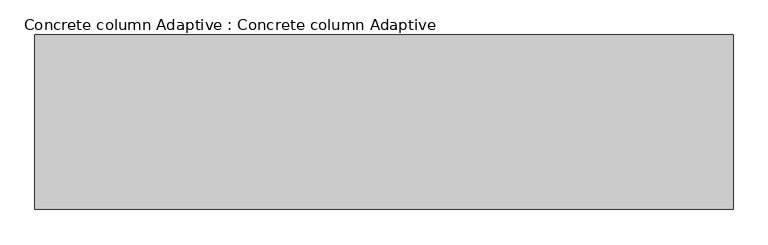
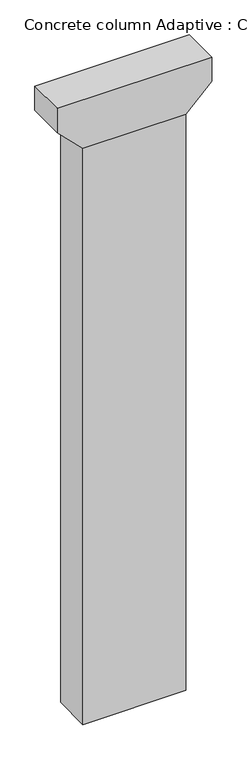
"""IFC4 building model written with IfcOpenShell, lengths in millimetres: proxy geometry, Concrete column Adaptive : Concrete column Adaptive."""

from ifc_helpers import new_model, si_unit, frame, origin, origin_with_axes, place, context, project, spatial, polyline, outline, extrude, source, transform, mapped, element, save


def concrete_column_adaptive_concrete_column_adaptive_fd02e230(model_context):
    return source(origin(), model_context, "Body", "SweptSolid", [
        extrude(outline(polyline([(51334.0, 6000.0), (51334.0, -6000.0), (49334.0, -6000.0), (47334.0, -4000.0), (47334.0, 4000.0), (49334.0, 6000.0), (51334.0, 6000.0)])), frame((0.0, -1500.0, 0.0), z_axis=(0.0, 1.0, 0.0), x_axis=(0.0, 0.0, 1.0)), (0.0, 0.0, 1.0), 3000.0),
        extrude(outline(polyline([(-4000.0, -1500.0), (-4000.0, 1500.0), (4000.0, 1500.0), (4000.0, -1500.0), (-4000.0, -1500.0)])), origin_with_axes(), (0.0, 0.0, 1.0), 47334.0),
    ])


if __name__ == "__main__":
    model = new_model("IFC4")
    model_context = context("Model", 3, world=origin())
    ifc_project = project(units=[si_unit("LENGTHUNIT", "METRE", prefix="MILLI")], contexts=[model_context])
    site = spatial("IfcSite", under=ifc_project)
    building = spatial("IfcBuilding", under=site)
    placement = place(None, origin())
    concrete_column_adaptive_concrete_column_adaptive_shape = concrete_column_adaptive_concrete_column_adaptive_fd02e230(model_context)
    element("IfcBuildingElementProxy", 1, Name="Concrete column Adaptive : Concrete column Adaptive", ObjectType="Concrete column Adaptive : Concrete column Adaptive", at=placement, inside=building, context=model_context, shape_type="MappedRepresentation", body=[
        mapped(concrete_column_adaptive_concrete_column_adaptive_shape, transform((0.0, 0.0, 0.0), x_axis=(1.0, 0.0, 0.0), y_axis=(0.0, 1.0, 0.0), z_axis=(0.0, 0.0, 1.0))),
    ])
    save(model, "model.ifc")

# Revit data of these elements
# Type "Concrete column Adaptive : Concrete column Adaptive"
#   Height [instance default] = 30000 mm
#   Default Elevation = 0
# Element 1 (IfcBuildingElementProxy, "Concrete column Adaptive : Concrete column Adaptive")
#   Height = 47334 mm
